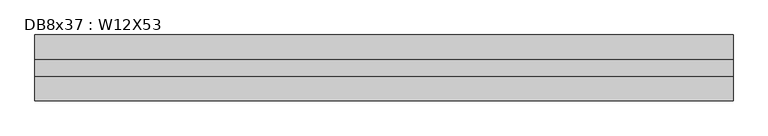
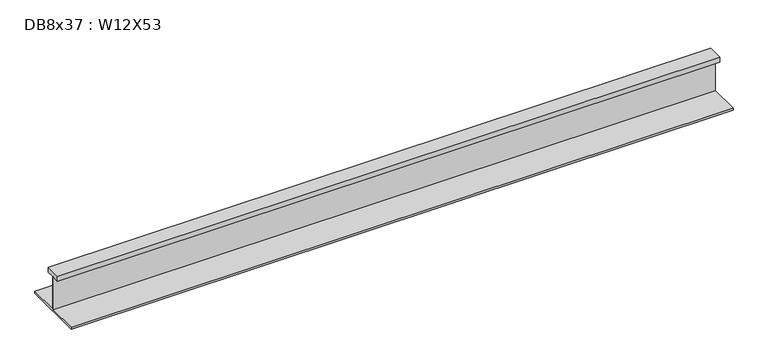
"""IFC4 building model written with IfcOpenShell, lengths in millimetres: beam geometry, DB8x37 : W12X53."""

from ifc_helpers import new_model, si_unit, frame, origin, place, context, project, spatial, polyline, outline, extrude, source, transform, mapped, element, save


def db8x37_w12x53_8e493c79(model_context):
    return source(origin(), model_context, "Body", "SweptSolid", [
        extrude(outline(polyline([(38.1, 145.415), (38.1, 120.015), (2.921, 120.015), (2.921, -48.4505), (152.4, -48.4505), (152.4, -58.1025), (-152.4, -58.1025), (-152.4, -48.4505), (-2.921, -48.4505), (-2.921, 120.015), (-38.1, 120.015), (-38.1, 145.415), (38.1, 145.415)])), frame((-1612.9, 0.0, 0.0), z_axis=(1.0, 0.0, 0.0), x_axis=(0.0, 1.0, 0.0)), (0.0, 0.0, 1.0), 3225.8),
    ])


if __name__ == "__main__":
    model = new_model("IFC4")
    model_context = context("Model", 3, world=origin())
    ifc_project = project(units=[si_unit("LENGTHUNIT", "METRE", prefix="MILLI")], contexts=[model_context])
    site = spatial("IfcSite", under=ifc_project)
    building = spatial("IfcBuilding", under=site)
    placement = place(None, origin())
    db8x37_w12x53_shape = db8x37_w12x53_8e493c79(model_context)
    element("IfcBeam", 1, ObjectType="DB8x37 : W12X53", at=placement, inside=building, context=model_context, shape_type="MappedRepresentation", body=[
        mapped(db8x37_w12x53_shape, transform((0.0, 0.0, 0.0), x_axis=(1.0, 0.0, 0.0), y_axis=(0.0, 1.0, 0.0), z_axis=(0.0, 0.0, 1.0))),
    ])
    save(model, "model.ifc")

# Revit data of these elements
# Type "DB8x37 : W12X53"
#   Assembly Code = "B10"
#   W = 53
#   Length [instance default] = 5' - 0"
#   bf = 0' - 10"
#   d = 1' - 0.1"
#   k = 0' - 1 3/8"
#   k2 = 0' - 0.8"
#   tf = 0' - 0.575"
#   tw = 0' - 0.345"
#   A = 0.108333 SF
#   Structural Material [instance default] = Steel ASTM A992
# Element 1 (IfcBeam, "DB8x37 : W12X53")
#   Materials on its faces: "Steel ASTM A992"
# Materials
#   "Steel ASTM A992": class "Metal", colour RGB 199 199 199, transparency 0, Description = "Structural steel 50ksi", Cost = 0
